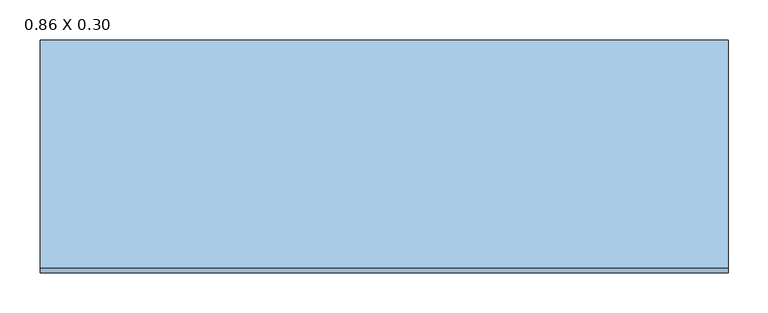
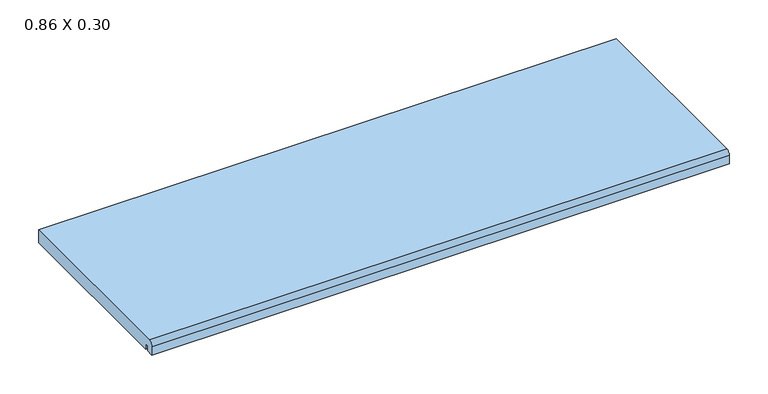
"""IFC4 building model written with IfcOpenShell, lengths in millimetres: window geometry, .CC_ND 300_PEDRA_PEITORIL RETO : 0.86 X 0.30."""

import ifcopenshell
import ifcopenshell.guid

model = None  # the IFC model being written
_history = None  # IfcOwnerHistory: only IFC2X3 demands one
_inside = {}  # id of a spatial element -> (the spatial element, [elements in it])
_under = {}  # id of a project, library or spatial element -> (it, [spatial elements below it])
_declared = {}  # id of a project -> (the project, [libraries it declares])
_typed = {}  # id of a type object -> (the type object, [elements of that type])
_made_of = {}  # id of a material, layer set ... -> (it, [elements and type objects made of it])


def new_model(schema):
    """Start an empty IFC model of exactly this schema.

    Asked for "IFC4X3", IfcOpenShell would pick the latest addendum, in which some entities
    have other attributes; the version numbers below select the first issue.
    IFC2X3 requires an IfcOwnerHistory on every rooted entity: one is made here for all.
    """
    global model, _history
    if schema == "IFC4X3":
        model = ifcopenshell.file(schema_version=(4, 3, 0, 0))
    else:
        model = ifcopenshell.file(schema=schema)
    _inside.clear()
    _under.clear()
    _declared.clear()
    _typed.clear()
    _made_of.clear()
    _history = None
    if model.schema == "IFC2X3":
        org = make("IfcOrganization", Name="unknown")
        user = make(
            "IfcPersonAndOrganization",
            ThePerson=make("IfcPerson", FamilyName="unknown"),
            TheOrganization=org,
        )
        app = make(
            "IfcApplication",
            ApplicationDeveloper=org,
            Version="unknown",
            ApplicationFullName="unknown",
            ApplicationIdentifier="unknown",
        )
        _history = make(
            "IfcOwnerHistory",
            OwningUser=user,
            OwningApplication=app,
            ChangeAction="ADDED",
            CreationDate=0,
        )
    return model


def make(cls, **values):
    """One entity of the class cls with the attributes given. An attribute that is None is left unset."""
    return model.create_entity(
        cls, **{name: value for name, value in values.items() if value is not None}
    )


def rooted(cls, **values):
    """An entity with a GlobalId (a new one), such as an element, a storey or a relation."""
    return make(cls, GlobalId=ifcopenshell.guid.new(), OwnerHistory=_history, **values)


def si_unit(unit_type, name, prefix=None):
    """IfcSIUnit, for example si_unit("LENGTHUNIT", "METRE", prefix="MILLI")."""
    return make("IfcSIUnit", UnitType=unit_type, Prefix=prefix, Name=name)


def assignment(units):
    """IfcUnitAssignment: the units of a project."""
    return None if units is None else make("IfcUnitAssignment", Units=units)


def point(xyz):
    """IfcCartesianPoint."""
    return None if xyz is None else make("IfcCartesianPoint", Coordinates=xyz)


def direction(xyz):
    """IfcDirection."""
    return None if xyz is None else make("IfcDirection", DirectionRatios=xyz)


def frame(location, z_axis=None, x_axis=None):
    """IfcAxis2Placement3D, a coordinate frame: its origin and axes. An axis left out is left unset."""
    return make(
        "IfcAxis2Placement3D",
        Location=point(location),
        Axis=direction(z_axis),
        RefDirection=direction(x_axis),
    )


def frame_2d(location, x_axis=None):
    """IfcAxis2Placement2D, a coordinate frame in the plane: its origin and x axis."""
    return make(
        "IfcAxis2Placement2D", Location=point(location), RefDirection=direction(x_axis)
    )


def origin():
    """The frame at (0, 0, 0) with its axes left unset."""
    return frame((0.0, 0.0, 0.0))


def place(relative_to, where):
    """IfcLocalPlacement: puts the frame where relative to a parent placement (None: the world)."""
    return make(
        "IfcLocalPlacement", PlacementRelTo=relative_to, RelativePlacement=where
    )


def context(
    kind, dimensions, precision=None, world=None, true_north=None, identifier=None
):
    """IfcGeometricRepresentationContext, for example the 3D "Model" context."""
    return make(
        "IfcGeometricRepresentationContext",
        ContextIdentifier=identifier,
        ContextType=kind,
        CoordinateSpaceDimension=dimensions,
        Precision=precision,
        WorldCoordinateSystem=world,
        TrueNorth=true_north,
    )


def project(units=None, contexts=None):
    """IfcProject with its units and contexts."""
    return rooted(
        "IfcProject",
        Name="project",
        RepresentationContexts=contexts,
        UnitsInContext=assignment(units),
    )


def spatial(cls, under=None, at=None, **own):
    """A site, building, storey or space (cls), placed at a placement, below another one or the project."""
    s = rooted(cls, ObjectPlacement=at, **own)
    if under is not None:
        _under.setdefault(under.id(), (under, []))[1].append(s)
    return s


def polyline(points):
    """IfcPolyline through the points."""
    return make("IfcPolyline", Points=[point(p) for p in points])


def circle_curve(where, radius):
    """IfcCircle in the frame where."""
    return make("IfcCircle", Position=where, Radius=radius)


def trimmed(basis, trim1, trim2, sense, master):
    """IfcTrimmedCurve: the piece of a basis curve between two trims."""
    return make(
        "IfcTrimmedCurve",
        BasisCurve=basis,
        Trim1=trim1,
        Trim2=trim2,
        SenseAgreement=sense,
        MasterRepresentation=master,
    )


def segment(curve, same_sense, transition):
    """IfcCompositeCurveSegment."""
    return make(
        "IfcCompositeCurveSegment",
        Transition=transition,
        SameSense=same_sense,
        ParentCurve=curve,
    )


def composite_curve(segments, self_intersect=None):
    """IfcCompositeCurve: segments joined end to end."""
    return make("IfcCompositeCurve", Segments=segments, SelfIntersect=self_intersect)


def outline(outer, holes=None, kind="AREA"):
    """IfcArbitraryClosedProfileDef: a profile drawn as a closed curve; with holes, ...WithVoids."""
    if holes is None:
        return make("IfcArbitraryClosedProfileDef", ProfileType=kind, OuterCurve=outer)
    return make(
        "IfcArbitraryProfileDefWithVoids",
        ProfileType=kind,
        OuterCurve=outer,
        InnerCurves=holes,
    )


def extrude(swept, where, along, depth):
    """IfcExtrudedAreaSolid: the profile swept, set in the frame where, extruded along a direction by depth."""
    return make(
        "IfcExtrudedAreaSolid",
        SweptArea=swept,
        Position=where,
        ExtrudedDirection=direction(along),
        Depth=depth,
    )


def shape(context_of_items, identifier, shape_type, items):
    """IfcShapeRepresentation: the items that make up one representation, for example the "Body"."""
    return make(
        "IfcShapeRepresentation",
        ContextOfItems=context_of_items,
        RepresentationIdentifier=identifier,
        RepresentationType=shape_type,
        Items=items,
    )


def source(mapping_origin, context_of_items, identifier, shape_type, items):
    """IfcRepresentationMap: a shape defined once, which mapped items show again and again."""
    return make(
        "IfcRepresentationMap",
        MappingOrigin=mapping_origin,
        MappedRepresentation=shape(context_of_items, identifier, shape_type, items),
    )


def transform(
    local_origin,
    x_axis=None,
    y_axis=None,
    z_axis=None,
    scale=None,
    scale2=None,
    scale3=None,
    uniform=True,
):
    """IfcCartesianTransformationOperator3D, or its non-uniform kind. x_axis, y_axis, z_axis: its Axis1, 2, 3."""
    if uniform:
        return make(
            "IfcCartesianTransformationOperator3D",
            Axis1=direction(x_axis),
            Axis2=direction(y_axis),
            LocalOrigin=point(local_origin),
            Scale=scale,
            Axis3=direction(z_axis),
        )
    return make(
        "IfcCartesianTransformationOperator3DnonUniform",
        Axis1=direction(x_axis),
        Axis2=direction(y_axis),
        LocalOrigin=point(local_origin),
        Scale=scale,
        Axis3=direction(z_axis),
        Scale2=scale2,
        Scale3=scale3,
    )


def mapped(mapping_source, mapping_target):
    """IfcMappedItem: shows the shape of a source again, moved by a transform."""
    return make(
        "IfcMappedItem", MappingSource=mapping_source, MappingTarget=mapping_target
    )


def made_of(thing, what):
    """Note that an element or type object is made of a material, layer set ...; save() writes the relation."""
    if what is not None:
        _made_of.setdefault(what.id(), (what, []))[1].append(thing)
    return thing


def element(
    cls,
    number,
    at=None,
    inside=None,
    cuts=None,
    type_object=None,
    material=None,
    context=None,
    identifier="Body",
    shape_type=None,
    held_by="IfcProductDefinitionShape",
    body=None,
    shapes=None,
    **own,
):
    """One element of the class cls, such as IfcWall. Its Tag is "e" and its number.

    at: its placement. inside: the storey or other place that contains it. cuts: it is an
    opening in that element (IfcRelVoidsElement). A single representation is given by context,
    identifier, shape_type and body (its items); several are given by shapes. held_by: the class
    of the entity that holds the representations. save() writes the other relations.
    """
    e = rooted(cls, Tag="e%d" % number, ObjectPlacement=at, **own)
    if body is not None:
        shapes = [shape(context, identifier, shape_type, body)]
    if shapes is not None:
        e.Representation = make(held_by, Representations=shapes)
    if inside is not None:
        _inside.setdefault(inside.id(), (inside, []))[1].append(e)
    if cuts is not None:
        rooted(
            "IfcRelVoidsElement", RelatingBuildingElement=cuts, RelatedOpeningElement=e
        )
    if type_object is not None:
        _typed.setdefault(type_object.id(), (type_object, []))[1].append(e)
    return made_of(e, material)


def aggregate(whole, parts):
    """IfcRelAggregates: a whole, such as a stair, and the parts it consists of."""
    return rooted("IfcRelAggregates", RelatingObject=whole, RelatedObjects=parts)


def save(model, path):
    """Write the relations noted so far, then the file.

    IfcRelAggregates (storeys below a building ...), IfcRelContainedInSpatialStructure (elements
    in a storey), IfcRelDefinesByType, IfcRelAssociatesMaterial and IfcRelDeclares: one each for
    every whole, place, type object, material and project.
    """
    for whole, parts in _under.values():
        aggregate(whole, parts)
    for where, things in _inside.values():
        rooted(
            "IfcRelContainedInSpatialStructure",
            RelatedElements=things,
            RelatingStructure=where,
        )
    for kind, things in _typed.values():
        rooted("IfcRelDefinesByType", RelatedObjects=things, RelatingType=kind)
    for what, things in _made_of.values():
        rooted("IfcRelAssociatesMaterial", RelatedObjects=things, RelatingMaterial=what)
    for by, libraries in _declared.values():
        rooted("IfcRelDeclares", RelatingContext=by, RelatedDefinitions=libraries)
    model.write(path)


def window_0_86_x_0_30_12272b82(model_context):
    return source(origin(), model_context, "Body", "SweptSolid", [
        extrude(outline(composite_curve([segment(polyline([(-132.5083081, 1480.0), (-132.5083081, 1488.1993124), (-137.2619526, 1488.1993124), (-137.2619526, 1480.0), (-148.0, 1480.0), (-148.0, 1493.3808343)]), True, "CONTINUOUS"), segment(trimmed(circle_curve(frame_2d((-141.3808343, 1493.3808343)), 6.6191657), [point((-148.0, 1493.3808343))], [point((-141.3808343, 1500.0))], False, "CARTESIAN"), True, "CONTINUOUS"), segment(polyline([(-141.3808343, 1500.0), (143.7, 1500.0), (143.7, 1480.0), (-132.5083081, 1480.0)]), True, "CONTINUOUS")], self_intersect=False)), frame((-430.0, 0.0, 0.0), z_axis=(1.0, 0.0, 0.0), x_axis=(0.0, 1.0, 0.0)), (0.0, 0.0, 1.0), 860.0),
    ])


if __name__ == "__main__":
    model = new_model("IFC4")
    model_context = context("Model", 3, world=origin())
    ifc_project = project(units=[si_unit("LENGTHUNIT", "METRE", prefix="MILLI")], contexts=[model_context])
    site = spatial("IfcSite", under=ifc_project)
    building = spatial("IfcBuilding", under=site)
    placement = place(None, origin())
    window_0_86_x_0_30_shape = window_0_86_x_0_30_12272b82(model_context)
    element("IfcWindow", 1, ObjectType=".CC_ND 300_PEDRA_PEITORIL RETO : 0.86 X 0.30", at=placement, inside=building, context=model_context, shape_type="MappedRepresentation", body=[
        mapped(window_0_86_x_0_30_shape, transform((0.0, 0.0, 0.0), x_axis=(1.0, 0.0, 0.0), y_axis=(0.0, 1.0, 0.0), z_axis=(0.0, 0.0, 1.0))),
    ])
    save(model, "model.ifc")

# Revit data of these elements
# Type ".CC_ND 300_PEDRA_PEITORIL RETO : 0.86 X 0.30"
#   Type Mark = "66"
#   Largura da pedra [instance default] = 0.26 m
#   Extensão interior peitoril [instance default] = 0.03 m
#   Extensão exterior peitoril [instance default] = 0.03 m
#   Espessura = 0.02 m
#   Comprimento = 0.86 m
#   Altura-padrão do peitoril = 1.48 m
#   Peitoril = .GRANITO_BRANCO_ITAUNAS
#   Rough Width = 0
#   Rough Height = 0
#   Height = 0
#   Wall Closure = (empty or 0)
#   Width = 0
# Element 1 (IfcWindow, ".CC_ND 300_PEDRA_PEITORIL RETO : 0.86 X 0.30")
#   Largura da pedra = 0.2917 m
#   Extensão interior peitoril = 0.0257 m
#   Materials on its faces: ".GRANITO_BRANCO_ITAUNAS"
# Materials
#   ".GRANITO_BRANCO_ITAUNAS": class ".CC_PEDRA REVEST.", colour RGB 202 195 174, transparency 0, Description = "Revestimento em granito", Cost = 0
